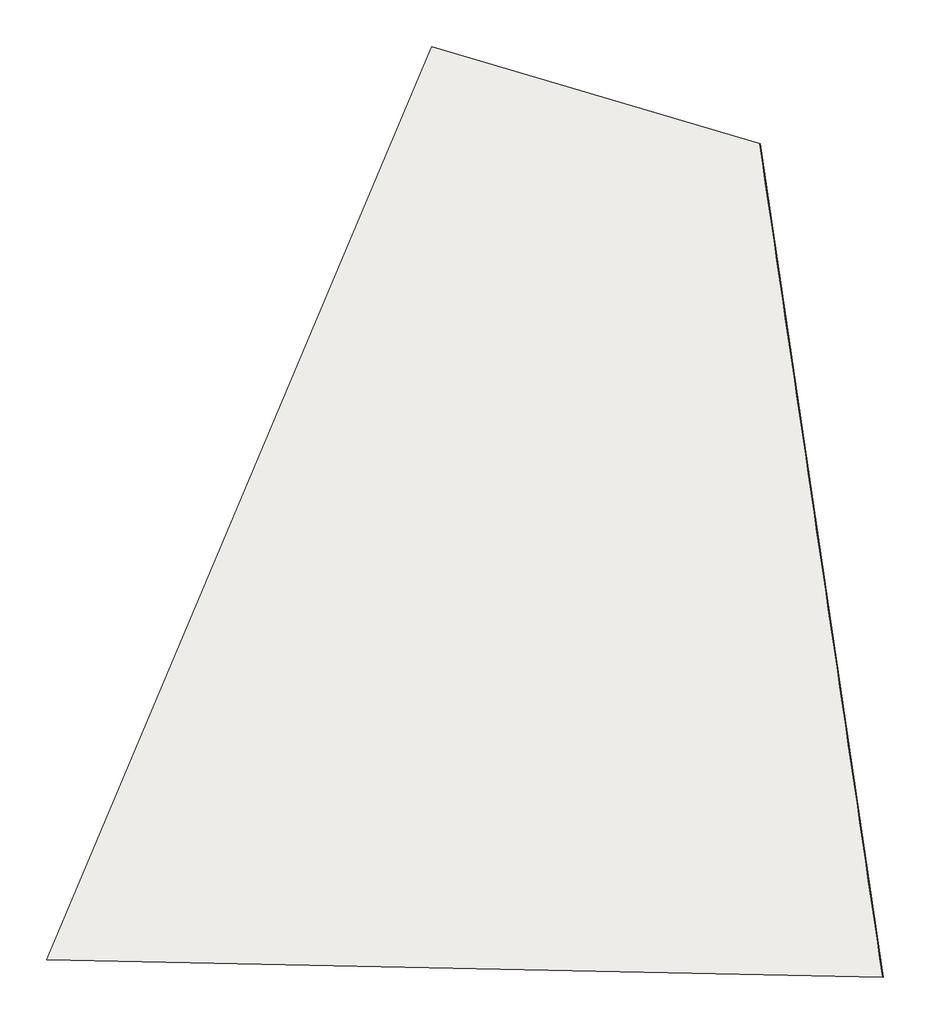
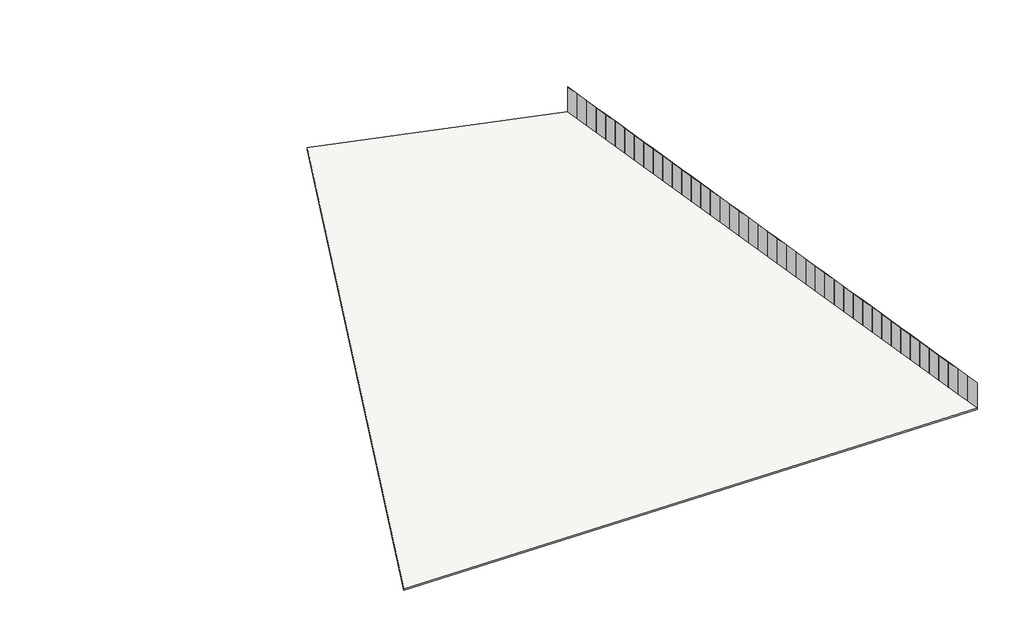
# One storey: 44 plates, 1 slab.
"""IFC4 building model written with IfcOpenShell, lengths in millimetres."""

import ifcopenshell
import ifcopenshell.guid

model = None  # the IFC model being written
_history = None  # IfcOwnerHistory: only IFC2X3 demands one
_inside = {}  # id of a spatial element -> (the spatial element, [elements in it])
_under = {}  # id of a project, library or spatial element -> (it, [spatial elements below it])
_declared = {}  # id of a project -> (the project, [libraries it declares])
_typed = {}  # id of a type object -> (the type object, [elements of that type])
_made_of = {}  # id of a material, layer set ... -> (it, [elements and type objects made of it])


def new_model(schema):
    """Start an empty IFC model of exactly this schema.

    Asked for "IFC4X3", IfcOpenShell would pick the latest addendum, in which some entities
    have other attributes; the version numbers below select the first issue.
    IFC2X3 requires an IfcOwnerHistory on every rooted entity: one is made here for all.
    """
    global model, _history
    if schema == "IFC4X3":
        model = ifcopenshell.file(schema_version=(4, 3, 0, 0))
    else:
        model = ifcopenshell.file(schema=schema)
    _inside.clear()
    _under.clear()
    _declared.clear()
    _typed.clear()
    _made_of.clear()
    _history = None
    if model.schema == "IFC2X3":
        org = make("IfcOrganization", Name="unknown")
        user = make(
            "IfcPersonAndOrganization",
            ThePerson=make("IfcPerson", FamilyName="unknown"),
            TheOrganization=org,
        )
        app = make(
            "IfcApplication",
            ApplicationDeveloper=org,
            Version="unknown",
            ApplicationFullName="unknown",
            ApplicationIdentifier="unknown",
        )
        _history = make(
            "IfcOwnerHistory",
            OwningUser=user,
            OwningApplication=app,
            ChangeAction="ADDED",
            CreationDate=0,
        )
    return model


def make(cls, **values):
    """One entity of the class cls with the attributes given. An attribute that is None is left unset."""
    return model.create_entity(
        cls, **{name: value for name, value in values.items() if value is not None}
    )


def rooted(cls, **values):
    """An entity with a GlobalId (a new one), such as an element, a storey or a relation."""
    return make(cls, GlobalId=ifcopenshell.guid.new(), OwnerHistory=_history, **values)


def si_unit(unit_type, name, prefix=None):
    """IfcSIUnit, for example si_unit("LENGTHUNIT", "METRE", prefix="MILLI")."""
    return make("IfcSIUnit", UnitType=unit_type, Prefix=prefix, Name=name)


def assignment(units):
    """IfcUnitAssignment: the units of a project."""
    return None if units is None else make("IfcUnitAssignment", Units=units)


def point(xyz):
    """IfcCartesianPoint."""
    return None if xyz is None else make("IfcCartesianPoint", Coordinates=xyz)


def direction(xyz):
    """IfcDirection."""
    return None if xyz is None else make("IfcDirection", DirectionRatios=xyz)


def frame(location, z_axis=None, x_axis=None):
    """IfcAxis2Placement3D, a coordinate frame: its origin and axes. An axis left out is left unset."""
    return make(
        "IfcAxis2Placement3D",
        Location=point(location),
        Axis=direction(z_axis),
        RefDirection=direction(x_axis),
    )


def origin():
    """The frame at (0, 0, 0) with its axes left unset."""
    return frame((0.0, 0.0, 0.0))


def origin_with_axes():
    """The frame at (0, 0, 0) with the z axis (0, 0, 1) and the x axis (1, 0, 0) written out."""
    return frame((0.0, 0.0, 0.0), z_axis=(0.0, 0.0, 1.0), x_axis=(1.0, 0.0, 0.0))


def place(relative_to, where):
    """IfcLocalPlacement: puts the frame where relative to a parent placement (None: the world)."""
    return make(
        "IfcLocalPlacement", PlacementRelTo=relative_to, RelativePlacement=where
    )


def context(
    kind, dimensions, precision=None, world=None, true_north=None, identifier=None
):
    """IfcGeometricRepresentationContext, for example the 3D "Model" context."""
    return make(
        "IfcGeometricRepresentationContext",
        ContextIdentifier=identifier,
        ContextType=kind,
        CoordinateSpaceDimension=dimensions,
        Precision=precision,
        WorldCoordinateSystem=world,
        TrueNorth=true_north,
    )


def project(units=None, contexts=None):
    """IfcProject with its units and contexts."""
    return rooted(
        "IfcProject",
        Name="project",
        RepresentationContexts=contexts,
        UnitsInContext=assignment(units),
    )


def spatial(cls, under=None, at=None, **own):
    """A site, building, storey or space (cls), placed at a placement, below another one or the project."""
    s = rooted(cls, ObjectPlacement=at, **own)
    if under is not None:
        _under.setdefault(under.id(), (under, []))[1].append(s)
    return s


def polyline(points):
    """IfcPolyline through the points."""
    return make("IfcPolyline", Points=[point(p) for p in points])


def outline(outer, holes=None, kind="AREA"):
    """IfcArbitraryClosedProfileDef: a profile drawn as a closed curve; with holes, ...WithVoids."""
    if holes is None:
        return make("IfcArbitraryClosedProfileDef", ProfileType=kind, OuterCurve=outer)
    return make(
        "IfcArbitraryProfileDefWithVoids",
        ProfileType=kind,
        OuterCurve=outer,
        InnerCurves=holes,
    )


def extrude(swept, where, along, depth):
    """IfcExtrudedAreaSolid: the profile swept, set in the frame where, extruded along a direction by depth."""
    return make(
        "IfcExtrudedAreaSolid",
        SweptArea=swept,
        Position=where,
        ExtrudedDirection=direction(along),
        Depth=depth,
    )


def shape(context_of_items, identifier, shape_type, items):
    """IfcShapeRepresentation: the items that make up one representation, for example the "Body"."""
    return make(
        "IfcShapeRepresentation",
        ContextOfItems=context_of_items,
        RepresentationIdentifier=identifier,
        RepresentationType=shape_type,
        Items=items,
    )


def source(mapping_origin, context_of_items, identifier, shape_type, items):
    """IfcRepresentationMap: a shape defined once, which mapped items show again and again."""
    return make(
        "IfcRepresentationMap",
        MappingOrigin=mapping_origin,
        MappedRepresentation=shape(context_of_items, identifier, shape_type, items),
    )


def transform(
    local_origin,
    x_axis=None,
    y_axis=None,
    z_axis=None,
    scale=None,
    scale2=None,
    scale3=None,
    uniform=True,
):
    """IfcCartesianTransformationOperator3D, or its non-uniform kind. x_axis, y_axis, z_axis: its Axis1, 2, 3."""
    if uniform:
        return make(
            "IfcCartesianTransformationOperator3D",
            Axis1=direction(x_axis),
            Axis2=direction(y_axis),
            LocalOrigin=point(local_origin),
            Scale=scale,
            Axis3=direction(z_axis),
        )
    return make(
        "IfcCartesianTransformationOperator3DnonUniform",
        Axis1=direction(x_axis),
        Axis2=direction(y_axis),
        LocalOrigin=point(local_origin),
        Scale=scale,
        Axis3=direction(z_axis),
        Scale2=scale2,
        Scale3=scale3,
    )


def mapped(mapping_source, mapping_target):
    """IfcMappedItem: shows the shape of a source again, moved by a transform."""
    return make(
        "IfcMappedItem", MappingSource=mapping_source, MappingTarget=mapping_target
    )


def made_of(thing, what):
    """Note that an element or type object is made of a material, layer set ...; save() writes the relation."""
    if what is not None:
        _made_of.setdefault(what.id(), (what, []))[1].append(thing)
    return thing


def element(
    cls,
    number,
    at=None,
    inside=None,
    cuts=None,
    type_object=None,
    material=None,
    context=None,
    identifier="Body",
    shape_type=None,
    held_by="IfcProductDefinitionShape",
    body=None,
    shapes=None,
    **own,
):
    """One element of the class cls, such as IfcWall. Its Tag is "e" and its number.

    at: its placement. inside: the storey or other place that contains it. cuts: it is an
    opening in that element (IfcRelVoidsElement). A single representation is given by context,
    identifier, shape_type and body (its items); several are given by shapes. held_by: the class
    of the entity that holds the representations. save() writes the other relations.
    """
    e = rooted(cls, Tag="e%d" % number, ObjectPlacement=at, **own)
    if body is not None:
        shapes = [shape(context, identifier, shape_type, body)]
    if shapes is not None:
        e.Representation = make(held_by, Representations=shapes)
    if inside is not None:
        _inside.setdefault(inside.id(), (inside, []))[1].append(e)
    if cuts is not None:
        rooted(
            "IfcRelVoidsElement", RelatingBuildingElement=cuts, RelatedOpeningElement=e
        )
    if type_object is not None:
        _typed.setdefault(type_object.id(), (type_object, []))[1].append(e)
    return made_of(e, material)


def aggregate(whole, parts):
    """IfcRelAggregates: a whole, such as a stair, and the parts it consists of."""
    return rooted("IfcRelAggregates", RelatingObject=whole, RelatedObjects=parts)


def save(model, path):
    """Write the relations noted so far, then the file.

    IfcRelAggregates (storeys below a building ...), IfcRelContainedInSpatialStructure (elements
    in a storey), IfcRelDefinesByType, IfcRelAssociatesMaterial and IfcRelDeclares: one each for
    every whole, place, type object, material and project.
    """
    for whole, parts in _under.values():
        aggregate(whole, parts)
    for where, things in _inside.values():
        rooted(
            "IfcRelContainedInSpatialStructure",
            RelatedElements=things,
            RelatingStructure=where,
        )
    for kind, things in _typed.values():
        rooted("IfcRelDefinesByType", RelatedObjects=things, RelatingType=kind)
    for what, things in _made_of.values():
        rooted("IfcRelAssociatesMaterial", RelatedObjects=things, RelatingMaterial=what)
    for by, libraries in _declared.values():
        rooted("IfcRelDeclares", RelatingContext=by, RelatedDefinitions=libraries)
    model.write(path)


def painel_do_sistema_1cdad03e(model_context):
    return source(origin(), model_context, "Body", "SweptSolid", [
        extrude(outline(polyline([(1500.0, 24.5), (-1500.0, 24.5), (-1500.0, 49.5), (1500.0, 49.5), (1500.0, 24.5)])), origin_with_axes(), (0.0, 0.0, 1.0), 1500.0),
    ])


def painel_do_sistema_1cb3a730(model_context):
    return source(origin(), model_context, "Body", "SweptSolid", [
        extrude(outline(polyline([(1500.0, 24.5), (-1500.0, 24.5), (-1500.0, 49.5), (1500.0, 49.5), (1500.0, 24.5)])), origin_with_axes(), (0.0, 0.0, 1.0), 20.0931032),
    ])


model = new_model("IFC4")

# Units and contexts
model_context = context("Model", 3, world=origin())
ifc_project = project(units=[si_unit("LENGTHUNIT", "METRE", prefix="MILLI")], contexts=[model_context])

# Site, building, storey
site = spatial("IfcSite", under=ifc_project)
building = spatial("IfcBuilding", under=site)
storey = spatial("IfcBuildingStorey", under=building, Name="Nível 8", Elevation=9000.0)

# Plates
placement = place(None, origin())
painel_do_sistema_shape = painel_do_sistema_1cdad03e(model_context)
element("IfcPlate", 1, ObjectType="Painel do sistema : Envidraçado", at=placement, inside=storey, context=model_context, shape_type="MappedRepresentation", body=[
    mapped(painel_do_sistema_shape, transform((27835.0106579, -36774.1442579, 10500.000015), x_axis=(0.0, 0.0, 1.0), y_axis=(-0.9892699032546327, -0.1460994815684493, 0.0), z_axis=(0.1460994815684493, -0.9892699032546327, 0.0))),
])
element("IfcPlate", 2, ObjectType="Painel do sistema : Envidraçado", at=placement, inside=storey, context=model_context, shape_type="MappedRepresentation", body=[
    mapped(painel_do_sistema_shape, transform((27615.8614356, -35290.239403, 10500.000015), x_axis=(0.0, 0.0, 1.0), y_axis=(-0.9892699032546328, -0.14609948156844887, 0.0), z_axis=(0.14609948156844887, -0.9892699032546328, 0.0))),
])
element("IfcPlate", 3, ObjectType="Painel do sistema : Envidraçado", at=placement, inside=storey, context=model_context, shape_type="MappedRepresentation", body=[
    mapped(painel_do_sistema_shape, transform((27396.7122132, -33806.3345481, 10500.000015), x_axis=(0.0, 0.0, 1.0), y_axis=(-0.9892699032546323, -0.1460994815684521, 0.0), z_axis=(0.1460994815684521, -0.9892699032546323, 0.0))),
])
element("IfcPlate", 4, ObjectType="Painel do sistema : Envidraçado", at=placement, inside=storey, context=model_context, shape_type="MappedRepresentation", body=[
    mapped(painel_do_sistema_shape, transform((27177.5629909, -32322.4296932, 10500.000015), x_axis=(0.0, 0.0, 1.0), y_axis=(-0.9892699032546327, -0.1460994815684493, 0.0), z_axis=(0.1460994815684493, -0.9892699032546327, 0.0))),
])
element("IfcPlate", 5, ObjectType="Painel do sistema : Envidraçado", at=placement, inside=storey, context=model_context, shape_type="MappedRepresentation", body=[
    mapped(painel_do_sistema_shape, transform((26958.4137685, -30838.5248383, 10500.000015), x_axis=(0.0, 0.0, 1.0), y_axis=(-0.9892699032546328, -0.1460994815684493, 0.0), z_axis=(0.1460994815684493, -0.9892699032546328, 0.0))),
])
element("IfcPlate", 6, ObjectType="Painel do sistema : Envidraçado", at=placement, inside=storey, context=model_context, shape_type="MappedRepresentation", body=[
    mapped(painel_do_sistema_shape, transform((26739.2645462, -29354.6199835, 10500.000015), x_axis=(0.0, 0.0, 1.0), y_axis=(-0.9892699032546323, -0.1460994815684521, 0.0), z_axis=(0.1460994815684521, -0.9892699032546323, 0.0))),
])
element("IfcPlate", 7, ObjectType="Painel do sistema : Envidraçado", at=placement, inside=storey, context=model_context, shape_type="MappedRepresentation", body=[
    mapped(painel_do_sistema_shape, transform((26520.1153238, -27870.7151286, 10500.000015), x_axis=(0.0, 0.0, 1.0), y_axis=(-0.9892699032546328, -0.14609948156844887, 0.0), z_axis=(0.14609948156844887, -0.9892699032546328, 0.0))),
])
element("IfcPlate", 8, ObjectType="Painel do sistema : Envidraçado", at=placement, inside=storey, context=model_context, shape_type="MappedRepresentation", body=[
    mapped(painel_do_sistema_shape, transform((26300.9661014, -26386.8102737, 10500.000015), x_axis=(0.0, 0.0, 1.0), y_axis=(-0.9892699032546328, -0.14609948156844926, 0.0), z_axis=(0.14609948156844926, -0.9892699032546328, 0.0))),
])
element("IfcPlate", 9, ObjectType="Painel do sistema : Envidraçado", at=placement, inside=storey, context=model_context, shape_type="MappedRepresentation", body=[
    mapped(painel_do_sistema_shape, transform((26081.8168791, -24902.9054188, 10500.000015), x_axis=(0.0, 0.0, 1.0), y_axis=(-0.9892699032546328, -0.14609948156844887, 0.0), z_axis=(0.14609948156844887, -0.9892699032546328, 0.0))),
])
element("IfcPlate", 10, ObjectType="Painel do sistema : Envidraçado", at=placement, inside=storey, context=model_context, shape_type="MappedRepresentation", body=[
    mapped(painel_do_sistema_shape, transform((25862.6676567, -23419.0005639, 10500.000015), x_axis=(0.0, 0.0, 1.0), y_axis=(-0.9892699032546328, -0.14609948156844887, 0.0), z_axis=(0.14609948156844887, -0.9892699032546328, 0.0))),
])
element("IfcPlate", 11, ObjectType="Painel do sistema : Envidraçado", at=placement, inside=storey, context=model_context, shape_type="MappedRepresentation", body=[
    mapped(painel_do_sistema_shape, transform((25643.5184344, -21935.095709, 10500.000015), x_axis=(0.0, 0.0, 1.0), y_axis=(-0.9892699032546328, -0.14609948156844926, 0.0), z_axis=(0.14609948156844926, -0.9892699032546328, 0.0))),
])
element("IfcPlate", 12, ObjectType="Painel do sistema : Envidraçado", at=placement, inside=storey, context=model_context, shape_type="MappedRepresentation", body=[
    mapped(painel_do_sistema_shape, transform((25424.369212, -20451.1908542, 10500.000015), x_axis=(0.0, 0.0, 1.0), y_axis=(-0.9892699032546319, -0.1460994815684545, 0.0), z_axis=(0.1460994815684545, -0.9892699032546319, 0.0))),
])
element("IfcPlate", 13, ObjectType="Painel do sistema : Envidraçado", at=placement, inside=storey, context=model_context, shape_type="MappedRepresentation", body=[
    mapped(painel_do_sistema_shape, transform((25205.2199897, -18967.2859993, 10500.000015), x_axis=(0.0, 0.0, 1.0), y_axis=(-0.9892699032546328, -0.14609948156844887, 0.0), z_axis=(0.14609948156844887, -0.9892699032546328, 0.0))),
])
element("IfcPlate", 14, ObjectType="Painel do sistema : Envidraçado", at=placement, inside=storey, context=model_context, shape_type="MappedRepresentation", body=[
    mapped(painel_do_sistema_shape, transform((24986.0707673, -17483.3811444, 10500.000015), x_axis=(0.0, 0.0, 1.0), y_axis=(-0.9892699032546328, -0.1460994815684491, 0.0), z_axis=(0.1460994815684491, -0.9892699032546328, 0.0))),
])
element("IfcPlate", 15, ObjectType="Painel do sistema : Envidraçado", at=placement, inside=storey, context=model_context, shape_type="MappedRepresentation", body=[
    mapped(painel_do_sistema_shape, transform((24766.921545, -15999.4762895, 10500.000015), x_axis=(0.0, 0.0, 1.0), y_axis=(-0.9892699032546328, -0.14609948156844926, 0.0), z_axis=(0.14609948156844926, -0.9892699032546328, 0.0))),
])
element("IfcPlate", 16, ObjectType="Painel do sistema : Envidraçado", at=placement, inside=storey, context=model_context, shape_type="MappedRepresentation", body=[
    mapped(painel_do_sistema_shape, transform((24547.7723226, -14515.5714346, 10500.000015), x_axis=(0.0, 0.0, 1.0), y_axis=(-0.9892699032546328, -0.14609948156844887, 0.0), z_axis=(0.14609948156844887, -0.9892699032546328, 0.0))),
])
element("IfcPlate", 17, ObjectType="Painel do sistema : Envidraçado", at=placement, inside=storey, context=model_context, shape_type="MappedRepresentation", body=[
    mapped(painel_do_sistema_shape, transform((24328.6231003, -13031.6665798, 10500.000015), x_axis=(0.0, 0.0, 1.0), y_axis=(-0.9892699032546323, -0.1460994815684521, 0.0), z_axis=(0.1460994815684521, -0.9892699032546323, 0.0))),
])
element("IfcPlate", 18, ObjectType="Painel do sistema : Envidraçado", at=placement, inside=storey, context=model_context, shape_type="MappedRepresentation", body=[
    mapped(painel_do_sistema_shape, transform((24109.4738779, -11547.7617249, 10500.000015), x_axis=(0.0, 0.0, 1.0), y_axis=(-0.9892699032546328, -0.1460994815684491, 0.0), z_axis=(0.1460994815684491, -0.9892699032546328, 0.0))),
])
element("IfcPlate", 19, ObjectType="Painel do sistema : Envidraçado", at=placement, inside=storey, context=model_context, shape_type="MappedRepresentation", body=[
    mapped(painel_do_sistema_shape, transform((23890.3246556, -10063.85687, 10500.000015), x_axis=(0.0, 0.0, 1.0), y_axis=(-0.9892699032546328, -0.14609948156844887, 0.0), z_axis=(0.14609948156844887, -0.9892699032546328, 0.0))),
])
element("IfcPlate", 20, ObjectType="Painel do sistema : Envidraçado", at=placement, inside=storey, context=model_context, shape_type="MappedRepresentation", body=[
    mapped(painel_do_sistema_shape, transform((23671.1754332, -8579.9520151, 10500.000015), x_axis=(0.0, 0.0, 1.0), y_axis=(-0.9892699032546328, -0.1460994815684491, 0.0), z_axis=(0.1460994815684491, -0.9892699032546328, 0.0))),
])
element("IfcPlate", 21, ObjectType="Painel do sistema : Envidraçado", at=placement, inside=storey, context=model_context, shape_type="MappedRepresentation", body=[
    mapped(painel_do_sistema_shape, transform((23452.0262109, -7096.0471602, 10500.000015), x_axis=(0.0, 0.0, 1.0), y_axis=(-0.9892699032546323, -0.1460994815684519, 0.0), z_axis=(0.1460994815684519, -0.9892699032546323, 0.0))),
])
element("IfcPlate", 22, ObjectType="Painel do sistema : Envidraçado", at=placement, inside=storey, context=model_context, shape_type="MappedRepresentation", body=[
    mapped(painel_do_sistema_shape, transform((23232.8769885, -5612.1423053, 10500.000015), x_axis=(0.0, 0.0, 1.0), y_axis=(-0.9892699032546328, -0.14609948156844926, 0.0), z_axis=(0.14609948156844926, -0.9892699032546328, 0.0))),
])
element("IfcPlate", 23, ObjectType="Painel do sistema : Envidraçado", at=placement, inside=storey, context=model_context, shape_type="MappedRepresentation", body=[
    mapped(painel_do_sistema_shape, transform((23013.7277662, -4128.2374505, 10500.000015), x_axis=(0.0, 0.0, 1.0), y_axis=(-0.9892699032546328, -0.14609948156844887, 0.0), z_axis=(0.14609948156844887, -0.9892699032546328, 0.0))),
])
element("IfcPlate", 24, ObjectType="Painel do sistema : Envidraçado", at=placement, inside=storey, context=model_context, shape_type="MappedRepresentation", body=[
    mapped(painel_do_sistema_shape, transform((22794.5785438, -2644.3325956, 10500.000015), x_axis=(0.0, 0.0, 1.0), y_axis=(-0.9892699032546324, -0.14609948156845148, 0.0), z_axis=(0.14609948156845148, -0.9892699032546324, 0.0))),
])
element("IfcPlate", 25, ObjectType="Painel do sistema : Envidraçado", at=placement, inside=storey, context=model_context, shape_type="MappedRepresentation", body=[
    mapped(painel_do_sistema_shape, transform((22575.4293215, -1160.4277407, 10500.000015), x_axis=(0.0, 0.0, 1.0), y_axis=(-0.9892699032546332, -0.14609948156844643, 0.0), z_axis=(0.14609948156844643, -0.9892699032546332, 0.0))),
])
element("IfcPlate", 26, ObjectType="Painel do sistema : Envidraçado", at=placement, inside=storey, context=model_context, shape_type="MappedRepresentation", body=[
    mapped(painel_do_sistema_shape, transform((22356.2800991, 323.4771142, 10500.000015), x_axis=(0.0, 0.0, 1.0), y_axis=(-0.9892699032546324, -0.1460994815684517, 0.0), z_axis=(0.1460994815684517, -0.9892699032546324, 0.0))),
])
element("IfcPlate", 27, ObjectType="Painel do sistema : Envidraçado", at=placement, inside=storey, context=model_context, shape_type="MappedRepresentation", body=[
    mapped(painel_do_sistema_shape, transform((22137.1308767, 1807.3819691, 10500.000015), x_axis=(0.0, 0.0, 1.0), y_axis=(-0.9892699032546327, -0.14609948156844949, 0.0), z_axis=(0.14609948156844949, -0.9892699032546327, 0.0))),
])
element("IfcPlate", 28, ObjectType="Painel do sistema : Envidraçado", at=placement, inside=storey, context=model_context, shape_type="MappedRepresentation", body=[
    mapped(painel_do_sistema_shape, transform((21917.9816544, 3291.2868239, 10500.000015), x_axis=(0.0, 0.0, 1.0), y_axis=(-0.9892699032546323, -0.1460994815684521, 0.0), z_axis=(0.1460994815684521, -0.9892699032546323, 0.0))),
])
element("IfcPlate", 29, ObjectType="Painel do sistema : Envidraçado", at=placement, inside=storey, context=model_context, shape_type="MappedRepresentation", body=[
    mapped(painel_do_sistema_shape, transform((21698.832432, 4775.1916788, 10500.000015), x_axis=(0.0, 0.0, 1.0), y_axis=(-0.9892699032546327, -0.14609948156844949, 0.0), z_axis=(0.14609948156844949, -0.9892699032546327, 0.0))),
])
element("IfcPlate", 30, ObjectType="Painel do sistema : Envidraçado", at=placement, inside=storey, context=model_context, shape_type="MappedRepresentation", body=[
    mapped(painel_do_sistema_shape, transform((21479.6832097, 6259.0965337, 10500.000015), x_axis=(0.0, 0.0, 1.0), y_axis=(-0.9892699032546328, -0.14609948156844926, 0.0), z_axis=(0.14609948156844926, -0.9892699032546328, 0.0))),
])
element("IfcPlate", 31, ObjectType="Painel do sistema : Envidraçado", at=placement, inside=storey, context=model_context, shape_type="MappedRepresentation", body=[
    mapped(painel_do_sistema_shape, transform((21260.5339873, 7743.0013886, 10500.000015), x_axis=(0.0, 0.0, 1.0), y_axis=(-0.9892699032546326, -0.14609948156844968, 0.0), z_axis=(0.14609948156844968, -0.9892699032546326, 0.0))),
])
element("IfcPlate", 32, ObjectType="Painel do sistema : Envidraçado", at=placement, inside=storey, context=model_context, shape_type="MappedRepresentation", body=[
    mapped(painel_do_sistema_shape, transform((21041.384765, 9226.9062435, 10500.000015), x_axis=(0.0, 0.0, 1.0), y_axis=(-0.9892699032546328, -0.14609948156844926, 0.0), z_axis=(0.14609948156844926, -0.9892699032546328, 0.0))),
])
element("IfcPlate", 33, ObjectType="Painel do sistema : Envidraçado", at=placement, inside=storey, context=model_context, shape_type="MappedRepresentation", body=[
    mapped(painel_do_sistema_shape, transform((20822.2355426, 10710.8110984, 10500.000015), x_axis=(0.0, 0.0, 1.0), y_axis=(-0.9892699032546328, -0.14609948156844926, 0.0), z_axis=(0.14609948156844926, -0.9892699032546328, 0.0))),
])
element("IfcPlate", 34, ObjectType="Painel do sistema : Envidraçado", at=placement, inside=storey, context=model_context, shape_type="MappedRepresentation", body=[
    mapped(painel_do_sistema_shape, transform((20603.0863203, 12194.7159532, 10500.000015), x_axis=(0.0, 0.0, 1.0), y_axis=(-0.9892699032546326, -0.1460994815684499, 0.0), z_axis=(0.1460994815684499, -0.9892699032546326, 0.0))),
])
element("IfcPlate", 35, ObjectType="Painel do sistema : Envidraçado", at=placement, inside=storey, context=model_context, shape_type="MappedRepresentation", body=[
    mapped(painel_do_sistema_shape, transform((20383.9370979, 13678.6208081, 10500.000015), x_axis=(0.0, 0.0, 1.0), y_axis=(-0.9892699032546326, -0.14609948156845054, 0.0), z_axis=(0.14609948156845054, -0.9892699032546326, 0.0))),
])
element("IfcPlate", 36, ObjectType="Painel do sistema : Envidraçado", at=placement, inside=storey, context=model_context, shape_type="MappedRepresentation", body=[
    mapped(painel_do_sistema_shape, transform((20164.7878756, 15162.525663, 10500.000015), x_axis=(0.0, 0.0, 1.0), y_axis=(-0.9892699032546328, -0.14609948156844887, 0.0), z_axis=(0.14609948156844887, -0.9892699032546328, 0.0))),
])
element("IfcPlate", 37, ObjectType="Painel do sistema : Envidraçado", at=placement, inside=storey, context=model_context, shape_type="MappedRepresentation", body=[
    mapped(painel_do_sistema_shape, transform((19945.6386532, 16646.4305179, 10500.000015), x_axis=(0.0, 0.0, 1.0), y_axis=(-0.9892699032546328, -0.14609948156844926, 0.0), z_axis=(0.14609948156844926, -0.9892699032546328, 0.0))),
])
element("IfcPlate", 38, ObjectType="Painel do sistema : Envidraçado", at=placement, inside=storey, context=model_context, shape_type="MappedRepresentation", body=[
    mapped(painel_do_sistema_shape, transform((19726.4894309, 18130.3353728, 10500.000015), x_axis=(0.0, 0.0, 1.0), y_axis=(-0.9892699032546326, -0.1460994815684501, 0.0), z_axis=(0.1460994815684501, -0.9892699032546326, 0.0))),
])
element("IfcPlate", 39, ObjectType="Painel do sistema : Envidraçado", at=placement, inside=storey, context=model_context, shape_type="MappedRepresentation", body=[
    mapped(painel_do_sistema_shape, transform((19507.3402085, 19614.2402276, 10500.000015), x_axis=(0.0, 0.0, 1.0), y_axis=(-0.9892699032546324, -0.1460994815684513, 0.0), z_axis=(0.1460994815684513, -0.9892699032546324, 0.0))),
])
element("IfcPlate", 40, ObjectType="Painel do sistema : Envidraçado", at=placement, inside=storey, context=model_context, shape_type="MappedRepresentation", body=[
    mapped(painel_do_sistema_shape, transform((19288.1909862, 21098.1450825, 10500.000015), x_axis=(0.0, 0.0, 1.0), y_axis=(-0.9892699032546326, -0.1460994815684501, 0.0), z_axis=(0.1460994815684501, -0.9892699032546326, 0.0))),
])
element("IfcPlate", 41, ObjectType="Painel do sistema : Envidraçado", at=placement, inside=storey, context=model_context, shape_type="MappedRepresentation", body=[
    mapped(painel_do_sistema_shape, transform((19069.0417638, 22582.0499374, 10500.000015), x_axis=(0.0, 0.0, 1.0), y_axis=(-0.9892699032546328, -0.14609948156844926, 0.0), z_axis=(0.14609948156844926, -0.9892699032546328, 0.0))),
])
element("IfcPlate", 42, ObjectType="Painel do sistema : Envidraçado", at=placement, inside=storey, context=model_context, shape_type="MappedRepresentation", body=[
    mapped(painel_do_sistema_shape, transform((18849.8925415, 24065.9547923, 10500.000015), x_axis=(0.0, 0.0, 1.0), y_axis=(-0.9892699032546326, -0.1460994815684501, 0.0), z_axis=(0.1460994815684501, -0.9892699032546326, 0.0))),
])
element("IfcPlate", 43, ObjectType="Painel do sistema : Envidraçado", at=placement, inside=storey, context=model_context, shape_type="MappedRepresentation", body=[
    mapped(painel_do_sistema_shape, transform((18630.7433191, 25549.8596472, 10500.000015), x_axis=(0.0, 0.0, 1.0), y_axis=(-0.9892699032546326, -0.14609948156844985, 0.0), z_axis=(0.14609948156844985, -0.9892699032546326, 0.0))),
])
painel_do_sistema_2_shape = painel_do_sistema_1cb3a730(model_context)
element("IfcPlate", 44, ObjectType="Painel do sistema : Envidraçado", at=placement, inside=storey, context=model_context, shape_type="MappedRepresentation", body=[
    mapped(painel_do_sistema_2_shape, transform((18627.8077271, 25569.7371494, 10500.000015), x_axis=(0.0, 0.0, 1.0), y_axis=(-0.9892699032546369, -0.14609948156842115, 0.0), z_axis=(0.14609948156842115, -0.9892699032546369, 0.0))),
])

# Slab
element("IfcSlab", 45, ObjectType="piso aula 04", at=placement, inside=storey, context=model_context, shape_type="SweptSolid", body=[
    extrude(outline(polyline([(18627.8077271, 25569.7371494), (28054.1598803, -38258.0491127), (-36012.0869489, -36912.3688141), (-6526.0277886, 32996.9225357), (18627.8077271, 25569.7371494)])), frame((0.0, 0.0, 8790.0), z_axis=(0.0, 0.0, 1.0), x_axis=(1.0, 0.0, 0.0)), (0.0, 0.0, 1.0), 210.0),
])

save(model, "model.ifc")

# Revit data of these elements
# Type "Painel do sistema : Envidraçado"
#   Construction Type Id = "GSP4R"
#   Analytic Construction = "Vidraça única Pilkington 1/8 pol"
#   Visual Light Transmittance = 0.9
#   Solar Heat Gain Coefficient = 0.86
#   Heat Transfer Coefficient (U) = 6.7069 W/(m²·K)
# Type "piso aula 04"
#   Function = 0
#   Layers, outside or top first: 0.02 m "Azulejo cerâmico" (function 4); 0.04 m "Concreto, Faixa de areia/cimento" (function 2); 0.15 m "Concreto,  Moldado in loco" (function 1)
# Elements 1, 2, 3, 4, 5, 6, 7, 8, 9, 10, 11, 12, 13, 14, 15, 16, 17, 18, 19, 20, 21, 22, 23, 24, 25, 26, 27, 28, 29, 30, 31, 32, 33, 34, 35, 36, 37, 38, 39, 40, 41, 42, 43, 44 (IfcPlate, "Painel do sistema : Envidraçado")
#   Phase Created = Construção nova
#   Materials on its faces: "Vidro"
# Element 45 (IfcSlab, "piso aula 04")
#   built-in parameter 1001955 = -0.287112 (stored number, unit not read)
#   Height Offset From Level = 0.00 m
#   Phase Created = Construção nova
#   Materials on its faces: "Concreto,  Moldado in loco", "Azulejo cerâmico"
# Materials
#   "Azulejo cerâmico": class "Cerâmica", colour RGB 246 230 196, transparency 0, Description = "Material físico", Cost = 0
#   "Concreto, Faixa de areia/cimento": class "Concreto", colour RGB 127 127 127, transparency 0, Description = "Revestimento de laje de concreto", Cost = 0
#   "Concreto,  Moldado in loco": class "Concreto", colour RGB 192 192 192, transparency 0, Description = "Material físico", Cost = 0
#   "Vidro": class "Vidro", colour RGB 0 128 192, transparency 0.9, Description = "Vidro de sílica", Cost = 0
